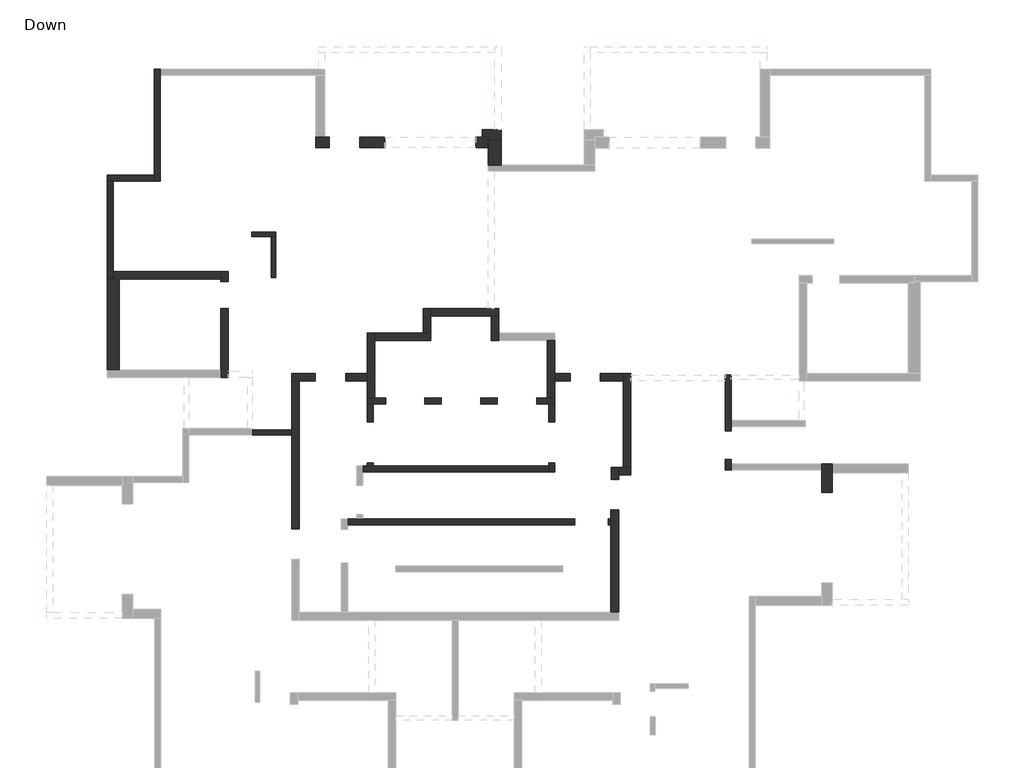
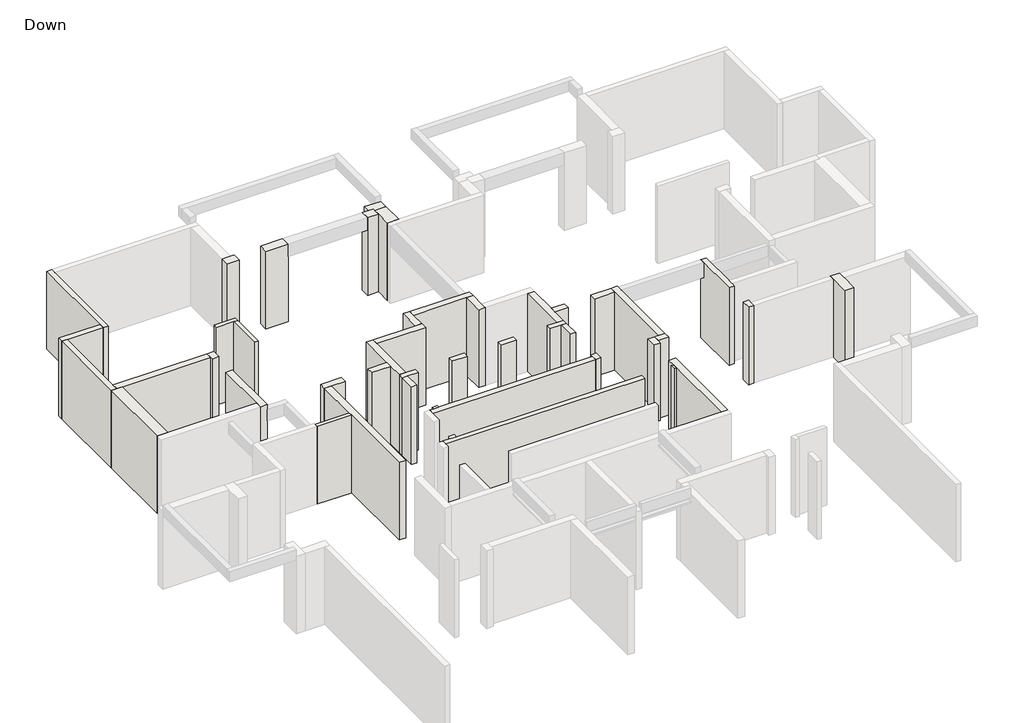
# One storey, part 2 of 3: 44 walls.
# Revit data of these elements (continued)
# Element 34 (IfcWall, "25") (continued)
#   SOFiSTiK_AMG_Comments = ""
#   Top Offset = 0 cm
#   Base Offset = 0 cm
#   wall height = 310 cm
#   SOFiSTiK_AMG_Scheduled = yes
#   SOFiSTiK_AMG_Adjusted = yes
#   Phase Created = New Construction
#   Base Constraint = Down
#   Top Constraint = Typical Floor
#   Materials on its faces: "Concrete"
# Element 35 (IfcWall, "25")
#   Comments = ""
#   Mark = "W88"
#   SOFiSTiK_EdgeZones = "W92"
#   SOFiSTiK_AMG_Comments = ""
#   Top Offset = 0 cm
#   Base Offset = 0 cm
#   wall height = 310 cm
#   SOFiSTiK_AMG_Scheduled = yes
#   SOFiSTiK_AMG_Adjusted = yes
#   Phase Created = New Construction
#   Base Constraint = Down
#   Top Constraint = Typical Floor
#   Materials on its faces: "Concrete"
# Element 36 (IfcWall, "25")
#   Comments = ""
#   Mark = "W89"
#   SOFiSTiK_EdgeZones = "W93"
#   SOFiSTiK_AMG_Comments = ""
#   Top Offset = 0 cm
#   Base Offset = 0 cm
#   wall height = 310 cm
#   SOFiSTiK_AMG_Scheduled = yes
#   SOFiSTiK_AMG_Adjusted = yes
#   Phase Created = New Construction
#   Base Constraint = Down
#   Top Constraint = Typical Floor
#   Materials on its faces: "Concrete"
# Element 37 (IfcWall, "25")
#   Comments = ""
#   Mark = "W91"
#   SOFiSTiK_EdgeZones = "W95"
#   SOFiSTiK_AMG_Comments = ""
#   Top Offset = 0 cm
#   Base Offset = 0 cm
#   wall height = 310 cm
#   SOFiSTiK_AMG_Scheduled = yes
#   SOFiSTiK_AMG_Adjusted = yes
#   Phase Created = New Construction
#   Base Constraint = Down
#   Top Constraint = Typical Floor
#   Materials on its faces: "Concrete"
# Element 38 (IfcWall, "35")
#   Comments = ""
#   Mark = "W49"
#   SOFiSTiK_EdgeZones = "W49"
#   SOFiSTiK_AMG_Comments = ""
#   Top Offset = 0 cm
#   Base Offset = 0 cm
#   wall height = 310 cm
#   SOFiSTiK_AMG_Scheduled = yes
#   SOFiSTiK_AMG_Adjusted = yes
#   Phase Created = New Construction
#   Base Constraint = Down
#   Top Constraint = Typical Floor
#   Materials on its faces: "Concrete"
# Element 39 (IfcWall, "35")
#   Comments = ""
#   Mark = "W50"
#   SOFiSTiK_EdgeZones = "W50"
#   SOFiSTiK_AMG_Comments = ""
#   Top Offset = 0 cm
#   Base Offset = 0 cm
#   wall height = 310 cm
#   SOFiSTiK_AMG_Scheduled = yes
#   SOFiSTiK_AMG_Adjusted = yes
#   Phase Created = New Construction
#   Base Constraint = Down
#   Top Constraint = Typical Floor
#   Materials on its faces: "Concrete"
# Element 40 (IfcWall, "35")
#   Comments = ""
#   Mark = "W54"
#   SOFiSTiK_EdgeZones = "W54"
#   SOFiSTiK_AMG_Comments = ""
#   Top Offset = 0 cm
#   Base Offset = 0 cm
#   wall height = 310 cm
#   SOFiSTiK_AMG_Scheduled = yes
#   SOFiSTiK_AMG_Adjusted = yes
#   Phase Created = New Construction
#   Base Constraint = Down
#   Top Constraint = Typical Floor
#   Materials on its faces: "Concrete"
# Element 41 (IfcWall, "35")
#   Comments = ""
#   Mark = "W59"
#   SOFiSTiK_EdgeZones = "W59"
#   SOFiSTiK_AMG_Comments = ""
#   Top Offset = 0 cm
#   Base Offset = 0 cm
#   wall height = 310 cm
#   SOFiSTiK_AMG_Scheduled = yes
#   SOFiSTiK_AMG_Adjusted = yes
#   Phase Created = New Construction
#   Base Constraint = Down
#   Top Constraint = Typical Floor
#   Materials on its faces: "Concrete"
# Element 42 (IfcWall, "35")
#   Comments = ""
#   Mark = "W60"
#   SOFiSTiK_EdgeZones = "W60"
#   SOFiSTiK_AMG_Comments = ""
#   Top Offset = 0 cm
#   Base Offset = 0 cm
#   wall height = 310 cm
#   SOFiSTiK_AMG_Scheduled = yes
#   SOFiSTiK_AMG_Adjusted = yes
#   Phase Created = New Construction
#   Base Constraint = Down
#   Top Constraint = Typical Floor
#   Materials on its faces: "Concrete"
# Element 43 (IfcWall, "40")
#   Comments = ""
#   Mark = "W96"
#   SOFiSTiK_EdgeZones = "W100"
#   SOFiSTiK_AMG_Comments = ""
#   Top Offset = 0 cm
#   Base Offset = 0 cm
#   wall height = 310 cm
#   SOFiSTiK_AMG_Scheduled = yes
#   SOFiSTiK_AMG_Adjusted = yes
#   Phase Created = New Construction
#   Base Constraint = Down
#   Top Constraint = Typical Floor
#   Materials on its faces: "Concrete"
# Element 44 (IfcWall, "42")
#   Comments = ""
#   Mark = "W111"
#   SOFiSTiK_EdgeZones = "W115"
#   SOFiSTiK_AMG_Comments = ""
#   Top Offset = 0 cm
#   Base Offset = 0 cm
#   wall height = 310 cm
#   SOFiSTiK_AMG_Scheduled = yes
#   SOFiSTiK_AMG_Adjusted = yes
#   Phase Created = New Construction
#   Base Constraint = Down
#   Top Constraint = Typical Floor
#   Materials on its faces: "Concrete"
# Materials
#   "Concrete": class "Concrete", colour RGB 192 192 192, transparency 0, Keynote = "01000", Description = "Cast-in-place concrete", Cost = 0
